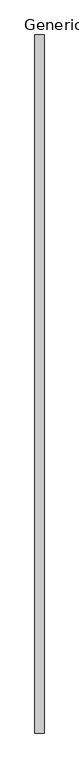
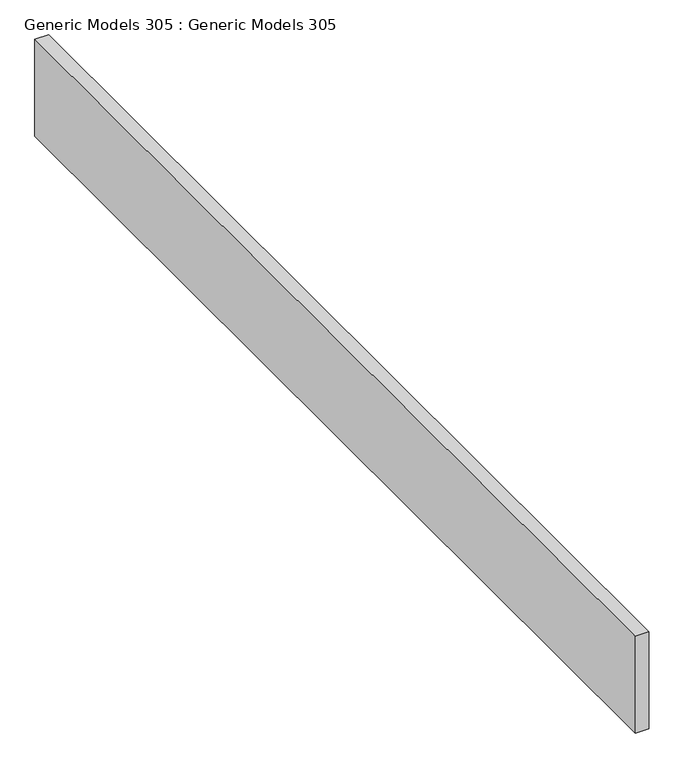
"""IFC4 building model written with IfcOpenShell, lengths in millimetres: proxy geometry, Generic Models 305 : Generic Models 305."""

import ifcopenshell
import ifcopenshell.guid

model = None  # the IFC model being written
_history = None  # IfcOwnerHistory: only IFC2X3 demands one
_inside = {}  # id of a spatial element -> (the spatial element, [elements in it])
_under = {}  # id of a project, library or spatial element -> (it, [spatial elements below it])
_declared = {}  # id of a project -> (the project, [libraries it declares])
_typed = {}  # id of a type object -> (the type object, [elements of that type])
_made_of = {}  # id of a material, layer set ... -> (it, [elements and type objects made of it])


def new_model(schema):
    """Start an empty IFC model of exactly this schema.

    Asked for "IFC4X3", IfcOpenShell would pick the latest addendum, in which some entities
    have other attributes; the version numbers below select the first issue.
    IFC2X3 requires an IfcOwnerHistory on every rooted entity: one is made here for all.
    """
    global model, _history
    if schema == "IFC4X3":
        model = ifcopenshell.file(schema_version=(4, 3, 0, 0))
    else:
        model = ifcopenshell.file(schema=schema)
    _inside.clear()
    _under.clear()
    _declared.clear()
    _typed.clear()
    _made_of.clear()
    _history = None
    if model.schema == "IFC2X3":
        org = make("IfcOrganization", Name="unknown")
        user = make(
            "IfcPersonAndOrganization",
            ThePerson=make("IfcPerson", FamilyName="unknown"),
            TheOrganization=org,
        )
        app = make(
            "IfcApplication",
            ApplicationDeveloper=org,
            Version="unknown",
            ApplicationFullName="unknown",
            ApplicationIdentifier="unknown",
        )
        _history = make(
            "IfcOwnerHistory",
            OwningUser=user,
            OwningApplication=app,
            ChangeAction="ADDED",
            CreationDate=0,
        )
    return model


def make(cls, **values):
    """One entity of the class cls with the attributes given. An attribute that is None is left unset."""
    return model.create_entity(
        cls, **{name: value for name, value in values.items() if value is not None}
    )


def rooted(cls, **values):
    """An entity with a GlobalId (a new one), such as an element, a storey or a relation."""
    return make(cls, GlobalId=ifcopenshell.guid.new(), OwnerHistory=_history, **values)


def si_unit(unit_type, name, prefix=None):
    """IfcSIUnit, for example si_unit("LENGTHUNIT", "METRE", prefix="MILLI")."""
    return make("IfcSIUnit", UnitType=unit_type, Prefix=prefix, Name=name)


def assignment(units):
    """IfcUnitAssignment: the units of a project."""
    return None if units is None else make("IfcUnitAssignment", Units=units)


def point(xyz):
    """IfcCartesianPoint."""
    return None if xyz is None else make("IfcCartesianPoint", Coordinates=xyz)


def direction(xyz):
    """IfcDirection."""
    return None if xyz is None else make("IfcDirection", DirectionRatios=xyz)


def frame(location, z_axis=None, x_axis=None):
    """IfcAxis2Placement3D, a coordinate frame: its origin and axes. An axis left out is left unset."""
    return make(
        "IfcAxis2Placement3D",
        Location=point(location),
        Axis=direction(z_axis),
        RefDirection=direction(x_axis),
    )


def origin():
    """The frame at (0, 0, 0) with its axes left unset."""
    return frame((0.0, 0.0, 0.0))


def place(relative_to, where):
    """IfcLocalPlacement: puts the frame where relative to a parent placement (None: the world)."""
    return make(
        "IfcLocalPlacement", PlacementRelTo=relative_to, RelativePlacement=where
    )


def context(
    kind, dimensions, precision=None, world=None, true_north=None, identifier=None
):
    """IfcGeometricRepresentationContext, for example the 3D "Model" context."""
    return make(
        "IfcGeometricRepresentationContext",
        ContextIdentifier=identifier,
        ContextType=kind,
        CoordinateSpaceDimension=dimensions,
        Precision=precision,
        WorldCoordinateSystem=world,
        TrueNorth=true_north,
    )


def project(units=None, contexts=None):
    """IfcProject with its units and contexts."""
    return rooted(
        "IfcProject",
        Name="project",
        RepresentationContexts=contexts,
        UnitsInContext=assignment(units),
    )


def spatial(cls, under=None, at=None, **own):
    """A site, building, storey or space (cls), placed at a placement, below another one or the project."""
    s = rooted(cls, ObjectPlacement=at, **own)
    if under is not None:
        _under.setdefault(under.id(), (under, []))[1].append(s)
    return s


def polyline(points):
    """IfcPolyline through the points."""
    return make("IfcPolyline", Points=[point(p) for p in points])


def outline(outer, holes=None, kind="AREA"):
    """IfcArbitraryClosedProfileDef: a profile drawn as a closed curve; with holes, ...WithVoids."""
    if holes is None:
        return make("IfcArbitraryClosedProfileDef", ProfileType=kind, OuterCurve=outer)
    return make(
        "IfcArbitraryProfileDefWithVoids",
        ProfileType=kind,
        OuterCurve=outer,
        InnerCurves=holes,
    )


def extrude(swept, where, along, depth):
    """IfcExtrudedAreaSolid: the profile swept, set in the frame where, extruded along a direction by depth."""
    return make(
        "IfcExtrudedAreaSolid",
        SweptArea=swept,
        Position=where,
        ExtrudedDirection=direction(along),
        Depth=depth,
    )


def shape(context_of_items, identifier, shape_type, items):
    """IfcShapeRepresentation: the items that make up one representation, for example the "Body"."""
    return make(
        "IfcShapeRepresentation",
        ContextOfItems=context_of_items,
        RepresentationIdentifier=identifier,
        RepresentationType=shape_type,
        Items=items,
    )


def source(mapping_origin, context_of_items, identifier, shape_type, items):
    """IfcRepresentationMap: a shape defined once, which mapped items show again and again."""
    return make(
        "IfcRepresentationMap",
        MappingOrigin=mapping_origin,
        MappedRepresentation=shape(context_of_items, identifier, shape_type, items),
    )


def transform(
    local_origin,
    x_axis=None,
    y_axis=None,
    z_axis=None,
    scale=None,
    scale2=None,
    scale3=None,
    uniform=True,
):
    """IfcCartesianTransformationOperator3D, or its non-uniform kind. x_axis, y_axis, z_axis: its Axis1, 2, 3."""
    if uniform:
        return make(
            "IfcCartesianTransformationOperator3D",
            Axis1=direction(x_axis),
            Axis2=direction(y_axis),
            LocalOrigin=point(local_origin),
            Scale=scale,
            Axis3=direction(z_axis),
        )
    return make(
        "IfcCartesianTransformationOperator3DnonUniform",
        Axis1=direction(x_axis),
        Axis2=direction(y_axis),
        LocalOrigin=point(local_origin),
        Scale=scale,
        Axis3=direction(z_axis),
        Scale2=scale2,
        Scale3=scale3,
    )


def mapped(mapping_source, mapping_target):
    """IfcMappedItem: shows the shape of a source again, moved by a transform."""
    return make(
        "IfcMappedItem", MappingSource=mapping_source, MappingTarget=mapping_target
    )


def made_of(thing, what):
    """Note that an element or type object is made of a material, layer set ...; save() writes the relation."""
    if what is not None:
        _made_of.setdefault(what.id(), (what, []))[1].append(thing)
    return thing


def element(
    cls,
    number,
    at=None,
    inside=None,
    cuts=None,
    type_object=None,
    material=None,
    context=None,
    identifier="Body",
    shape_type=None,
    held_by="IfcProductDefinitionShape",
    body=None,
    shapes=None,
    **own,
):
    """One element of the class cls, such as IfcWall. Its Tag is "e" and its number.

    at: its placement. inside: the storey or other place that contains it. cuts: it is an
    opening in that element (IfcRelVoidsElement). A single representation is given by context,
    identifier, shape_type and body (its items); several are given by shapes. held_by: the class
    of the entity that holds the representations. save() writes the other relations.
    """
    e = rooted(cls, Tag="e%d" % number, ObjectPlacement=at, **own)
    if body is not None:
        shapes = [shape(context, identifier, shape_type, body)]
    if shapes is not None:
        e.Representation = make(held_by, Representations=shapes)
    if inside is not None:
        _inside.setdefault(inside.id(), (inside, []))[1].append(e)
    if cuts is not None:
        rooted(
            "IfcRelVoidsElement", RelatingBuildingElement=cuts, RelatedOpeningElement=e
        )
    if type_object is not None:
        _typed.setdefault(type_object.id(), (type_object, []))[1].append(e)
    return made_of(e, material)


def aggregate(whole, parts):
    """IfcRelAggregates: a whole, such as a stair, and the parts it consists of."""
    return rooted("IfcRelAggregates", RelatingObject=whole, RelatedObjects=parts)


def save(model, path):
    """Write the relations noted so far, then the file.

    IfcRelAggregates (storeys below a building ...), IfcRelContainedInSpatialStructure (elements
    in a storey), IfcRelDefinesByType, IfcRelAssociatesMaterial and IfcRelDeclares: one each for
    every whole, place, type object, material and project.
    """
    for whole, parts in _under.values():
        aggregate(whole, parts)
    for where, things in _inside.values():
        rooted(
            "IfcRelContainedInSpatialStructure",
            RelatedElements=things,
            RelatingStructure=where,
        )
    for kind, things in _typed.values():
        rooted("IfcRelDefinesByType", RelatedObjects=things, RelatingType=kind)
    for what, things in _made_of.values():
        rooted("IfcRelAssociatesMaterial", RelatedObjects=things, RelatingMaterial=what)
    for by, libraries in _declared.values():
        rooted("IfcRelDeclares", RelatingContext=by, RelatedDefinitions=libraries)
    model.write(path)


def generic_models_305_generic_models_305_818cdebe(model_context):
    return source(origin(), model_context, "Body", "SweptSolid", [
        extrude(outline(polyline([(4902.0263704, -311.7230338), (4863.9263704, -311.7230338), (4863.9263704, 2596.5769662), (4902.0263704, 2596.5769662), (4902.0263704, -311.7230338)])), frame((0.0, 0.0, 129247.646), z_axis=(0.0, 0.0, 1.0), x_axis=(1.0, 0.0, 0.0)), (0.0, 0.0, 1.0), 285.75),
    ])


if __name__ == "__main__":
    model = new_model("IFC4")
    model_context = context("Model", 3, world=origin())
    ifc_project = project(units=[si_unit("LENGTHUNIT", "METRE", prefix="MILLI")], contexts=[model_context])
    site = spatial("IfcSite", under=ifc_project)
    building = spatial("IfcBuilding", under=site)
    placement = place(None, origin())
    generic_models_305_generic_models_305_shape = generic_models_305_generic_models_305_818cdebe(model_context)
    element("IfcBuildingElementProxy", 1, Name="Generic Models 305 : Generic Models 305", ObjectType="Generic Models 305 : Generic Models 305", at=placement, inside=building, context=model_context, shape_type="MappedRepresentation", body=[
        mapped(generic_models_305_generic_models_305_shape, transform((0.0, 0.0, 0.0), x_axis=(1.0, 0.0, 0.0), y_axis=(0.0, 1.0, 0.0), z_axis=(0.0, 0.0, 1.0))),
    ])
    save(model, "model.ifc")

# Revit data of these elements
# Element 1 (IfcBuildingElementProxy, "Generic Models 305 : Generic Models 305")
#   Materials on its faces: "_STRUCTURAL MEMBER (SEE STRUCT. DWGS)"
# Materials
#   "_STRUCTURAL MEMBER (SEE STRUCT. DWGS)": class "Generic", colour RGB 209 182 141, transparency 0, Cost = 0
